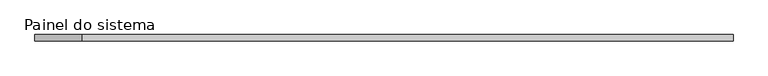
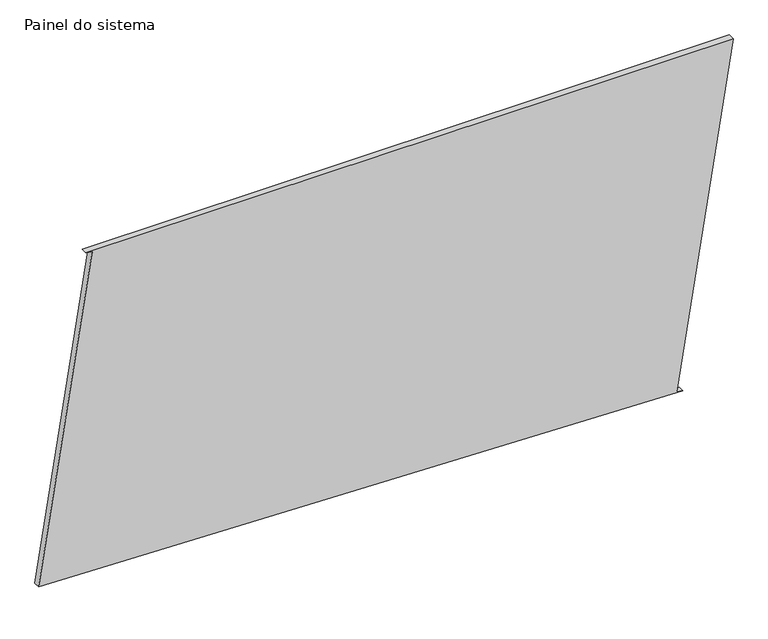
"""IFC4 building model written with IfcOpenShell, lengths in millimetres: plate geometry, Painel do sistema : Envidraçado."""

from ifc_helpers import new_model, si_unit, frame, origin, place, context, project, spatial, polyline, outline, extrude, source, transform, mapped, element, save


def painel_do_sistema_008d99d4(model_context):
    return source(origin(), model_context, "Body", "SweptSolid", [
        extrude(outline(polyline([(0.0, 1183.9950583), (3.9380954, 1159.3071786), (1414.0819772, 1384.2467497), (1414.0819772, -1195.5909756), (1410.1438818, -1170.9030959), (72.6946874, -1384.2467497), (0.0, 1183.9950583)])), frame((0.0, 24.5, 0.0), z_axis=(0.0, 1.0, 0.0), x_axis=(0.0, 0.0, 1.0)), (0.0, 0.0, 1.0), 25.0),
    ])


if __name__ == "__main__":
    model = new_model("IFC4")
    model_context = context("Model", 3, world=origin())
    ifc_project = project(units=[si_unit("LENGTHUNIT", "METRE", prefix="MILLI")], contexts=[model_context])
    site = spatial("IfcSite", under=ifc_project)
    building = spatial("IfcBuilding", under=site)
    placement = place(None, origin())
    painel_do_sistema_shape = painel_do_sistema_008d99d4(model_context)
    element("IfcPlate", 1, ObjectType="Painel do sistema : Envidraçado", at=placement, inside=building, context=model_context, shape_type="MappedRepresentation", body=[
        mapped(painel_do_sistema_shape, transform((0.0, 0.0, 0.0), x_axis=(1.0, 0.0, 0.0), y_axis=(0.0, 1.0, 0.0), z_axis=(0.0, 0.0, 1.0))),
    ])
    save(model, "model.ifc")

# Revit data of these elements
# Type "Painel do sistema : Envidraçado"
#   Construction Type Id = "GSP4R"
#   Analytic Construction = "Vidraça única Pilkington 1/8 pol"
#   Visual Light Transmittance = 0.9
#   Solar Heat Gain Coefficient = 0.86
#   Heat Transfer Coefficient (U) = 6.7069 W/(m²·K)
# Element 1 (IfcPlate, "Painel do sistema : Envidraçado")
#   Materials on its faces: "Vidro"
# Materials
#   "Vidro": class "Vidro", colour RGB 0 128 192, transparency 0.9, Description = "Vidro de sílica", Cost = 0
